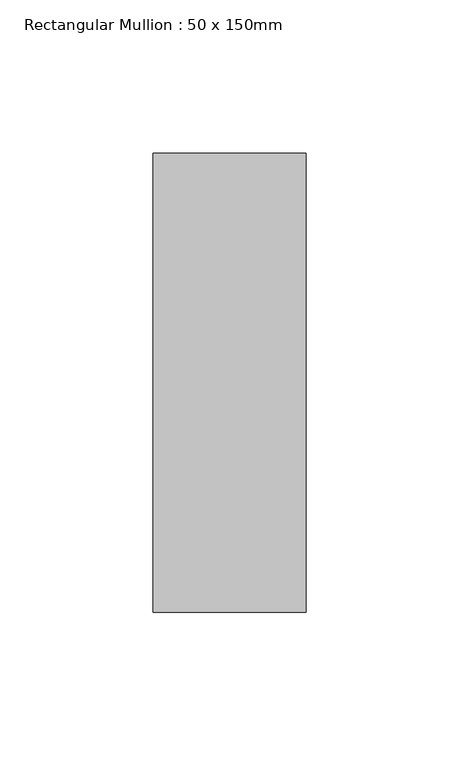
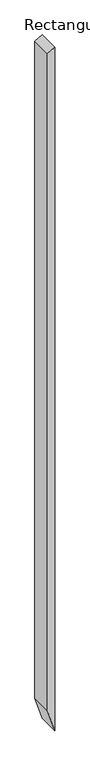
"""IFC4 building model written with IfcOpenShell, lengths in millimetres: member geometry, Rectangular Mullion : 50 x 150mm."""

import ifcopenshell
import ifcopenshell.guid

model = None  # the IFC model being written
_history = None  # IfcOwnerHistory: only IFC2X3 demands one
_inside = {}  # id of a spatial element -> (the spatial element, [elements in it])
_under = {}  # id of a project, library or spatial element -> (it, [spatial elements below it])
_declared = {}  # id of a project -> (the project, [libraries it declares])
_typed = {}  # id of a type object -> (the type object, [elements of that type])
_made_of = {}  # id of a material, layer set ... -> (it, [elements and type objects made of it])


def new_model(schema):
    """Start an empty IFC model of exactly this schema.

    Asked for "IFC4X3", IfcOpenShell would pick the latest addendum, in which some entities
    have other attributes; the version numbers below select the first issue.
    IFC2X3 requires an IfcOwnerHistory on every rooted entity: one is made here for all.
    """
    global model, _history
    if schema == "IFC4X3":
        model = ifcopenshell.file(schema_version=(4, 3, 0, 0))
    else:
        model = ifcopenshell.file(schema=schema)
    _inside.clear()
    _under.clear()
    _declared.clear()
    _typed.clear()
    _made_of.clear()
    _history = None
    if model.schema == "IFC2X3":
        org = make("IfcOrganization", Name="unknown")
        user = make(
            "IfcPersonAndOrganization",
            ThePerson=make("IfcPerson", FamilyName="unknown"),
            TheOrganization=org,
        )
        app = make(
            "IfcApplication",
            ApplicationDeveloper=org,
            Version="unknown",
            ApplicationFullName="unknown",
            ApplicationIdentifier="unknown",
        )
        _history = make(
            "IfcOwnerHistory",
            OwningUser=user,
            OwningApplication=app,
            ChangeAction="ADDED",
            CreationDate=0,
        )
    return model


def make(cls, **values):
    """One entity of the class cls with the attributes given. An attribute that is None is left unset."""
    return model.create_entity(
        cls, **{name: value for name, value in values.items() if value is not None}
    )


def rooted(cls, **values):
    """An entity with a GlobalId (a new one), such as an element, a storey or a relation."""
    return make(cls, GlobalId=ifcopenshell.guid.new(), OwnerHistory=_history, **values)


def si_unit(unit_type, name, prefix=None):
    """IfcSIUnit, for example si_unit("LENGTHUNIT", "METRE", prefix="MILLI")."""
    return make("IfcSIUnit", UnitType=unit_type, Prefix=prefix, Name=name)


def assignment(units):
    """IfcUnitAssignment: the units of a project."""
    return None if units is None else make("IfcUnitAssignment", Units=units)


def point(xyz):
    """IfcCartesianPoint."""
    return None if xyz is None else make("IfcCartesianPoint", Coordinates=xyz)


def direction(xyz):
    """IfcDirection."""
    return None if xyz is None else make("IfcDirection", DirectionRatios=xyz)


def frame(location, z_axis=None, x_axis=None):
    """IfcAxis2Placement3D, a coordinate frame: its origin and axes. An axis left out is left unset."""
    return make(
        "IfcAxis2Placement3D",
        Location=point(location),
        Axis=direction(z_axis),
        RefDirection=direction(x_axis),
    )


def origin():
    """The frame at (0, 0, 0) with its axes left unset."""
    return frame((0.0, 0.0, 0.0))


def place(relative_to, where):
    """IfcLocalPlacement: puts the frame where relative to a parent placement (None: the world)."""
    return make(
        "IfcLocalPlacement", PlacementRelTo=relative_to, RelativePlacement=where
    )


def context(
    kind, dimensions, precision=None, world=None, true_north=None, identifier=None
):
    """IfcGeometricRepresentationContext, for example the 3D "Model" context."""
    return make(
        "IfcGeometricRepresentationContext",
        ContextIdentifier=identifier,
        ContextType=kind,
        CoordinateSpaceDimension=dimensions,
        Precision=precision,
        WorldCoordinateSystem=world,
        TrueNorth=true_north,
    )


def project(units=None, contexts=None):
    """IfcProject with its units and contexts."""
    return rooted(
        "IfcProject",
        Name="project",
        RepresentationContexts=contexts,
        UnitsInContext=assignment(units),
    )


def spatial(cls, under=None, at=None, **own):
    """A site, building, storey or space (cls), placed at a placement, below another one or the project."""
    s = rooted(cls, ObjectPlacement=at, **own)
    if under is not None:
        _under.setdefault(under.id(), (under, []))[1].append(s)
    return s


def polyline(points):
    """IfcPolyline through the points."""
    return make("IfcPolyline", Points=[point(p) for p in points])


def outline(outer, holes=None, kind="AREA"):
    """IfcArbitraryClosedProfileDef: a profile drawn as a closed curve; with holes, ...WithVoids."""
    if holes is None:
        return make("IfcArbitraryClosedProfileDef", ProfileType=kind, OuterCurve=outer)
    return make(
        "IfcArbitraryProfileDefWithVoids",
        ProfileType=kind,
        OuterCurve=outer,
        InnerCurves=holes,
    )


def extrude(swept, where, along, depth):
    """IfcExtrudedAreaSolid: the profile swept, set in the frame where, extruded along a direction by depth."""
    return make(
        "IfcExtrudedAreaSolid",
        SweptArea=swept,
        Position=where,
        ExtrudedDirection=direction(along),
        Depth=depth,
    )


def shape(context_of_items, identifier, shape_type, items):
    """IfcShapeRepresentation: the items that make up one representation, for example the "Body"."""
    return make(
        "IfcShapeRepresentation",
        ContextOfItems=context_of_items,
        RepresentationIdentifier=identifier,
        RepresentationType=shape_type,
        Items=items,
    )


def source(mapping_origin, context_of_items, identifier, shape_type, items):
    """IfcRepresentationMap: a shape defined once, which mapped items show again and again."""
    return make(
        "IfcRepresentationMap",
        MappingOrigin=mapping_origin,
        MappedRepresentation=shape(context_of_items, identifier, shape_type, items),
    )


def transform(
    local_origin,
    x_axis=None,
    y_axis=None,
    z_axis=None,
    scale=None,
    scale2=None,
    scale3=None,
    uniform=True,
):
    """IfcCartesianTransformationOperator3D, or its non-uniform kind. x_axis, y_axis, z_axis: its Axis1, 2, 3."""
    if uniform:
        return make(
            "IfcCartesianTransformationOperator3D",
            Axis1=direction(x_axis),
            Axis2=direction(y_axis),
            LocalOrigin=point(local_origin),
            Scale=scale,
            Axis3=direction(z_axis),
        )
    return make(
        "IfcCartesianTransformationOperator3DnonUniform",
        Axis1=direction(x_axis),
        Axis2=direction(y_axis),
        LocalOrigin=point(local_origin),
        Scale=scale,
        Axis3=direction(z_axis),
        Scale2=scale2,
        Scale3=scale3,
    )


def mapped(mapping_source, mapping_target):
    """IfcMappedItem: shows the shape of a source again, moved by a transform."""
    return make(
        "IfcMappedItem", MappingSource=mapping_source, MappingTarget=mapping_target
    )


def made_of(thing, what):
    """Note that an element or type object is made of a material, layer set ...; save() writes the relation."""
    if what is not None:
        _made_of.setdefault(what.id(), (what, []))[1].append(thing)
    return thing


def element(
    cls,
    number,
    at=None,
    inside=None,
    cuts=None,
    type_object=None,
    material=None,
    context=None,
    identifier="Body",
    shape_type=None,
    held_by="IfcProductDefinitionShape",
    body=None,
    shapes=None,
    **own,
):
    """One element of the class cls, such as IfcWall. Its Tag is "e" and its number.

    at: its placement. inside: the storey or other place that contains it. cuts: it is an
    opening in that element (IfcRelVoidsElement). A single representation is given by context,
    identifier, shape_type and body (its items); several are given by shapes. held_by: the class
    of the entity that holds the representations. save() writes the other relations.
    """
    e = rooted(cls, Tag="e%d" % number, ObjectPlacement=at, **own)
    if body is not None:
        shapes = [shape(context, identifier, shape_type, body)]
    if shapes is not None:
        e.Representation = make(held_by, Representations=shapes)
    if inside is not None:
        _inside.setdefault(inside.id(), (inside, []))[1].append(e)
    if cuts is not None:
        rooted(
            "IfcRelVoidsElement", RelatingBuildingElement=cuts, RelatedOpeningElement=e
        )
    if type_object is not None:
        _typed.setdefault(type_object.id(), (type_object, []))[1].append(e)
    return made_of(e, material)


def aggregate(whole, parts):
    """IfcRelAggregates: a whole, such as a stair, and the parts it consists of."""
    return rooted("IfcRelAggregates", RelatingObject=whole, RelatedObjects=parts)


def save(model, path):
    """Write the relations noted so far, then the file.

    IfcRelAggregates (storeys below a building ...), IfcRelContainedInSpatialStructure (elements
    in a storey), IfcRelDefinesByType, IfcRelAssociatesMaterial and IfcRelDeclares: one each for
    every whole, place, type object, material and project.
    """
    for whole, parts in _under.values():
        aggregate(whole, parts)
    for where, things in _inside.values():
        rooted(
            "IfcRelContainedInSpatialStructure",
            RelatedElements=things,
            RelatingStructure=where,
        )
    for kind, things in _typed.values():
        rooted("IfcRelDefinesByType", RelatedObjects=things, RelatingType=kind)
    for what, things in _made_of.values():
        rooted("IfcRelAssociatesMaterial", RelatedObjects=things, RelatingMaterial=what)
    for by, libraries in _declared.values():
        rooted("IfcRelDeclares", RelatingContext=by, RelatedDefinitions=libraries)
    model.write(path)


def rectangular_mullion_50_x_150mm_460fb724(model_context):
    return source(origin(), model_context, "Body", "SweptSolid", [
        extrude(outline(polyline([(0.0, 0.0), (-29.3010691, -50.0), (-4821.4590794, -50.0), (-4983.1907154, 0.0), (0.0, 0.0)])), frame((0.0, -75.0, 0.0), z_axis=(0.0, 1.0, 0.0), x_axis=(0.0, 0.0, 1.0)), (0.0, 0.0, 1.0), 150.0),
    ])


if __name__ == "__main__":
    model = new_model("IFC4")
    model_context = context("Model", 3, world=origin())
    ifc_project = project(units=[si_unit("LENGTHUNIT", "METRE", prefix="MILLI")], contexts=[model_context])
    site = spatial("IfcSite", under=ifc_project)
    building = spatial("IfcBuilding", under=site)
    placement = place(None, origin())
    rectangular_mullion_50_x_150mm_shape = rectangular_mullion_50_x_150mm_460fb724(model_context)
    element("IfcMember", 1, ObjectType="Rectangular Mullion : 50 x 150mm", at=placement, inside=building, context=model_context, shape_type="MappedRepresentation", body=[
        mapped(rectangular_mullion_50_x_150mm_shape, transform((0.0, 0.0, 0.0), x_axis=(1.0, 0.0, 0.0), y_axis=(0.0, 1.0, 0.0), z_axis=(0.0, 0.0, 1.0))),
    ])
    save(model, "model.ifc")

# Revit data of these elements
# Type "Rectangular Mullion : 50 x 150mm"
#   built-in parameter 1007304 = 0.492126 (stored number, unit not read)
#   built-in parameter 1007301 = 0.082021 (stored number, unit not read)
#   built-in parameter 1007300 = 0.082021 (stored number, unit not read)
# Element 1 (IfcMember, "Rectangular Mullion : 50 x 150mm")
#   Materials on its faces: "Metal - Aluminium"
# Materials
#   "Metal - Aluminium": class "Metal", colour RGB 247 247 247, transparency 0
